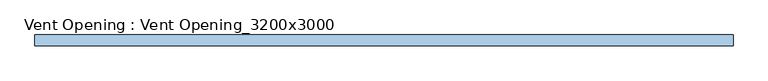
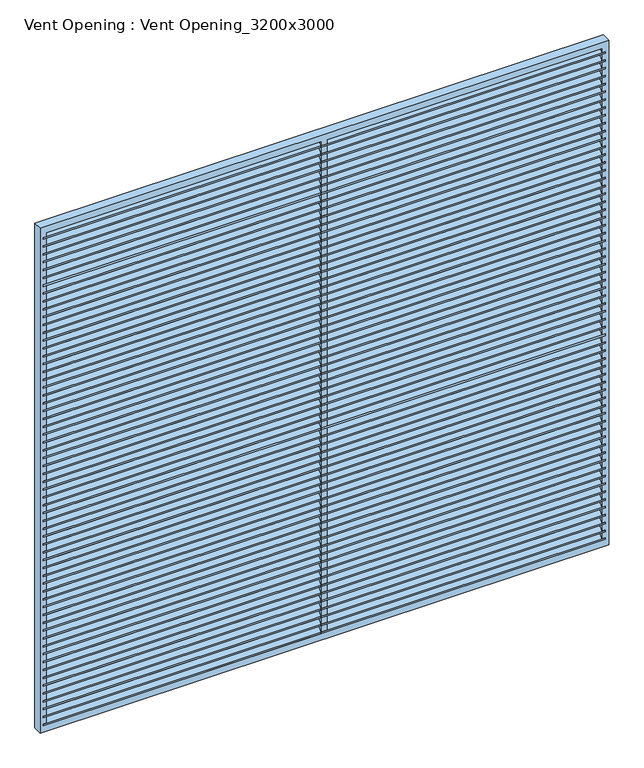
"""IFC4 building model written with IfcOpenShell, lengths in millimetres: window geometry, Vent Opening : Vent Opening_3200x3000."""

from ifc_helpers import new_model, si_unit, frame, origin, place, context, project, spatial, polyline, outline, extrude, source, transform, mapped, element, save


def vent_opening_vent_opening_3200x3000_4c487494(model_context):
    return source(origin(), model_context, "Body", "SweptSolid", [
        extrude(outline(polyline([(118.65, 3390.2900041), (118.65, 3381.309748), (93.65, 3406.309748), (68.65, 3381.309748), (68.65, 3390.2900041), (93.65, 3415.2900041), (118.65, 3390.2900041)])), frame((-1580.95, 0.0, 0.0), z_axis=(1.0, 0.0, 0.0), x_axis=(0.0, 1.0, 0.0)), (0.0, 0.0, 1.0), 3161.9),
        extrude(outline(polyline([(118.65, 3343.6800083), (118.65, 3334.6997521), (93.65, 3359.6997521), (68.65, 3334.6997521), (68.65, 3343.6800083), (93.65, 3368.6800083), (118.65, 3343.6800083)])), frame((-1580.95, 0.0, 0.0), z_axis=(1.0, 0.0, 0.0), x_axis=(0.0, 1.0, 0.0)), (0.0, 0.0, 1.0), 3161.9),
        extrude(outline(polyline([(118.65, 3297.0700124), (118.65, 3288.0897563), (93.65, 3313.0897563), (68.65, 3288.0897563), (68.65, 3297.0700124), (93.65, 3322.0700124), (118.65, 3297.0700124)])), frame((-1580.95, 0.0, 0.0), z_axis=(1.0, 0.0, 0.0), x_axis=(0.0, 1.0, 0.0)), (0.0, 0.0, 1.0), 3161.9),
        extrude(outline(polyline([(118.65, 3250.4600165), (118.65, 3241.4797604), (93.65, 3266.4797604), (68.65, 3241.4797604), (68.65, 3250.4600165), (93.65, 3275.4600165), (118.65, 3250.4600165)])), frame((-1580.95, 0.0, 0.0), z_axis=(1.0, 0.0, 0.0), x_axis=(0.0, 1.0, 0.0)), (0.0, 0.0, 1.0), 3161.9),
        extrude(outline(polyline([(118.65, 3203.8500207), (118.65, 3194.8697645), (93.65, 3219.8697645), (68.65, 3194.8697645), (68.65, 3203.8500207), (93.65, 3228.8500207), (118.65, 3203.8500207)])), frame((-1580.95, 0.0, 0.0), z_axis=(1.0, 0.0, 0.0), x_axis=(0.0, 1.0, 0.0)), (0.0, 0.0, 1.0), 3161.9),
        extrude(outline(polyline([(118.65, 3157.2400248), (118.65, 3148.2597687), (93.65, 3173.2597687), (68.65, 3148.2597687), (68.65, 3157.2400248), (93.65, 3182.2400248), (118.65, 3157.2400248)])), frame((-1580.95, 0.0, 0.0), z_axis=(1.0, 0.0, 0.0), x_axis=(0.0, 1.0, 0.0)), (0.0, 0.0, 1.0), 3161.9),
        extrude(outline(polyline([(118.65, 3110.6300289), (118.65, 3101.6497728), (93.65, 3126.6497728), (68.65, 3101.6497728), (68.65, 3110.6300289), (93.65, 3135.6300289), (118.65, 3110.6300289)])), frame((-1580.95, 0.0, 0.0), z_axis=(1.0, 0.0, 0.0), x_axis=(0.0, 1.0, 0.0)), (0.0, 0.0, 1.0), 3161.9),
        extrude(outline(polyline([(118.65, 3064.020033), (118.65, 3055.0397769), (93.65, 3080.0397769), (68.65, 3055.0397769), (68.65, 3064.020033), (93.65, 3089.020033), (118.65, 3064.020033)])), frame((-1580.95, 0.0, 0.0), z_axis=(1.0, 0.0, 0.0), x_axis=(0.0, 1.0, 0.0)), (0.0, 0.0, 1.0), 3161.9),
        extrude(outline(polyline([(118.65, 3017.4100372), (118.65, 3008.4297811), (93.65, 3033.4297811), (68.65, 3008.4297811), (68.65, 3017.4100372), (93.65, 3042.4100372), (118.65, 3017.4100372)])), frame((-1580.95, 0.0, 0.0), z_axis=(1.0, 0.0, 0.0), x_axis=(0.0, 1.0, 0.0)), (0.0, 0.0, 1.0), 3161.9),
        extrude(outline(polyline([(118.65, 2970.8000413), (118.65, 2961.8197852), (93.65, 2986.8197852), (68.65, 2961.8197852), (68.65, 2970.8000413), (93.65, 2995.8000413), (118.65, 2970.8000413)])), frame((-1580.95, 0.0, 0.0), z_axis=(1.0, 0.0, 0.0), x_axis=(0.0, 1.0, 0.0)), (0.0, 0.0, 1.0), 3161.9),
        extrude(outline(polyline([(118.65, 2924.1900454), (118.65, 2915.2097893), (93.65, 2940.2097893), (68.65, 2915.2097893), (68.65, 2924.1900454), (93.65, 2949.1900454), (118.65, 2924.1900454)])), frame((-1580.95, 0.0, 0.0), z_axis=(1.0, 0.0, 0.0), x_axis=(0.0, 1.0, 0.0)), (0.0, 0.0, 1.0), 3161.9),
        extrude(outline(polyline([(118.65, 2877.5800496), (118.65, 2868.5997935), (93.65, 2893.5997935), (68.65, 2868.5997935), (68.65, 2877.5800496), (93.65, 2902.5800496), (118.65, 2877.5800496)])), frame((-1580.95, 0.0, 0.0), z_axis=(1.0, 0.0, 0.0), x_axis=(0.0, 1.0, 0.0)), (0.0, 0.0, 1.0), 3161.9),
        extrude(outline(polyline([(118.65, 2830.9700537), (118.65, 2821.9897976), (93.65, 2846.9897976), (68.65, 2821.9897976), (68.65, 2830.9700537), (93.65, 2855.9700537), (118.65, 2830.9700537)])), frame((-1580.95, 0.0, 0.0), z_axis=(1.0, 0.0, 0.0), x_axis=(0.0, 1.0, 0.0)), (0.0, 0.0, 1.0), 3161.9),
        extrude(outline(polyline([(118.65, 2784.3600578), (118.65, 2775.3798017), (93.65, 2800.3798017), (68.65, 2775.3798017), (68.65, 2784.3600578), (93.65, 2809.3600578), (118.65, 2784.3600578)])), frame((-1580.95, 0.0, 0.0), z_axis=(1.0, 0.0, 0.0), x_axis=(0.0, 1.0, 0.0)), (0.0, 0.0, 1.0), 3161.9),
        extrude(outline(polyline([(118.65, 2737.750062), (118.65, 2728.7698058), (93.65, 2753.7698058), (68.65, 2728.7698058), (68.65, 2737.750062), (93.65, 2762.750062), (118.65, 2737.750062)])), frame((-1580.95, 0.0, 0.0), z_axis=(1.0, 0.0, 0.0), x_axis=(0.0, 1.0, 0.0)), (0.0, 0.0, 1.0), 3161.9),
        extrude(outline(polyline([(118.65, 2691.1400661), (118.65, 2682.15981), (93.65, 2707.15981), (68.65, 2682.15981), (68.65, 2691.1400661), (93.65, 2716.1400661), (118.65, 2691.1400661)])), frame((-1580.95, 0.0, 0.0), z_axis=(1.0, 0.0, 0.0), x_axis=(0.0, 1.0, 0.0)), (0.0, 0.0, 1.0), 3161.9),
        extrude(outline(polyline([(118.65, 2644.5300702), (118.65, 2635.5498141), (93.65, 2660.5498141), (68.65, 2635.5498141), (68.65, 2644.5300702), (93.65, 2669.5300702), (118.65, 2644.5300702)])), frame((-1580.95, 0.0, 0.0), z_axis=(1.0, 0.0, 0.0), x_axis=(0.0, 1.0, 0.0)), (0.0, 0.0, 1.0), 3161.9),
        extrude(outline(polyline([(118.65, 2597.9200744), (118.65, 2588.9398182), (93.65, 2613.9398182), (68.65, 2588.9398182), (68.65, 2597.9200744), (93.65, 2622.9200744), (118.65, 2597.9200744)])), frame((-1580.95, 0.0, 0.0), z_axis=(1.0, 0.0, 0.0), x_axis=(0.0, 1.0, 0.0)), (0.0, 0.0, 1.0), 3161.9),
        extrude(outline(polyline([(118.65, 2551.3100785), (118.65, 2542.3298224), (93.65, 2567.3298224), (68.65, 2542.3298224), (68.65, 2551.3100785), (93.65, 2576.3100785), (118.65, 2551.3100785)])), frame((-1580.95, 0.0, 0.0), z_axis=(1.0, 0.0, 0.0), x_axis=(0.0, 1.0, 0.0)), (0.0, 0.0, 1.0), 3161.9),
        extrude(outline(polyline([(118.65, 2504.7000826), (118.65, 2495.7198265), (93.65, 2520.7198265), (68.65, 2495.7198265), (68.65, 2504.7000826), (93.65, 2529.7000826), (118.65, 2504.7000826)])), frame((-1580.95, 0.0, 0.0), z_axis=(1.0, 0.0, 0.0), x_axis=(0.0, 1.0, 0.0)), (0.0, 0.0, 1.0), 3161.9),
        extrude(outline(polyline([(118.65, 2458.0900868), (118.65, 2449.1098306), (93.65, 2474.1098306), (68.65, 2449.1098306), (68.65, 2458.0900868), (93.65, 2483.0900868), (118.65, 2458.0900868)])), frame((-1580.95, 0.0, 0.0), z_axis=(1.0, 0.0, 0.0), x_axis=(0.0, 1.0, 0.0)), (0.0, 0.0, 1.0), 3161.9),
        extrude(outline(polyline([(118.65, 2411.4800909), (118.65, 2402.4998348), (93.65, 2427.4998348), (68.65, 2402.4998348), (68.65, 2411.4800909), (93.65, 2436.4800909), (118.65, 2411.4800909)])), frame((-1580.95, 0.0, 0.0), z_axis=(1.0, 0.0, 0.0), x_axis=(0.0, 1.0, 0.0)), (0.0, 0.0, 1.0), 3161.9),
        extrude(outline(polyline([(118.65, 2364.870095), (118.65, 2355.8898389), (93.65, 2380.8898389), (68.65, 2355.8898389), (68.65, 2364.870095), (93.65, 2389.870095), (118.65, 2364.870095)])), frame((-1580.95, 0.0, 0.0), z_axis=(1.0, 0.0, 0.0), x_axis=(0.0, 1.0, 0.0)), (0.0, 0.0, 1.0), 3161.9),
        extrude(outline(polyline([(118.65, 2318.2600991), (118.65, 2309.279843), (93.65, 2334.279843), (68.65, 2309.279843), (68.65, 2318.2600991), (93.65, 2343.2600991), (118.65, 2318.2600991)])), frame((-1580.95, 0.0, 0.0), z_axis=(1.0, 0.0, 0.0), x_axis=(0.0, 1.0, 0.0)), (0.0, 0.0, 1.0), 3161.9),
        extrude(outline(polyline([(118.65, 2271.6501033), (118.65, 2262.6698472), (93.65, 2287.6698472), (68.65, 2262.6698472), (68.65, 2271.6501033), (93.65, 2296.6501033), (118.65, 2271.6501033)])), frame((-1580.95, 0.0, 0.0), z_axis=(1.0, 0.0, 0.0), x_axis=(0.0, 1.0, 0.0)), (0.0, 0.0, 1.0), 3161.9),
        extrude(outline(polyline([(118.65, 2225.0401074), (118.65, 2216.0598513), (93.65, 2241.0598513), (68.65, 2216.0598513), (68.65, 2225.0401074), (93.65, 2250.0401074), (118.65, 2225.0401074)])), frame((-1580.95, 0.0, 0.0), z_axis=(1.0, 0.0, 0.0), x_axis=(0.0, 1.0, 0.0)), (0.0, 0.0, 1.0), 3161.9),
        extrude(outline(polyline([(118.65, 2178.4301115), (118.65, 2169.4498554), (93.65, 2194.4498554), (68.65, 2169.4498554), (68.65, 2178.4301115), (93.65, 2203.4301115), (118.65, 2178.4301115)])), frame((-1580.95, 0.0, 0.0), z_axis=(1.0, 0.0, 0.0), x_axis=(0.0, 1.0, 0.0)), (0.0, 0.0, 1.0), 3161.9),
        extrude(outline(polyline([(118.65, 2131.8201157), (118.65, 2122.8398595), (93.65, 2147.8398595), (68.65, 2122.8398595), (68.65, 2131.8201157), (93.65, 2156.8201157), (118.65, 2131.8201157)])), frame((-1580.95, 0.0, 0.0), z_axis=(1.0, 0.0, 0.0), x_axis=(0.0, 1.0, 0.0)), (0.0, 0.0, 1.0), 3161.9),
        extrude(outline(polyline([(118.65, 2085.2101198), (118.65, 2076.2298637), (93.65, 2101.2298637), (68.65, 2076.2298637), (68.65, 2085.2101198), (93.65, 2110.2101198), (118.65, 2085.2101198)])), frame((-1580.95, 0.0, 0.0), z_axis=(1.0, 0.0, 0.0), x_axis=(0.0, 1.0, 0.0)), (0.0, 0.0, 1.0), 3161.9),
        extrude(outline(polyline([(118.65, 2038.6001239), (118.65, 2029.6198678), (93.65, 2054.6198678), (68.65, 2029.6198678), (68.65, 2038.6001239), (93.65, 2063.6001239), (118.65, 2038.6001239)])), frame((-1580.95, 0.0, 0.0), z_axis=(1.0, 0.0, 0.0), x_axis=(0.0, 1.0, 0.0)), (0.0, 0.0, 1.0), 3161.9),
        extrude(outline(polyline([(118.65, 1991.9901281), (118.65, 1983.0098719), (93.65, 2008.0098719), (68.65, 1983.0098719), (68.65, 1991.9901281), (93.65, 2016.9901281), (118.65, 1991.9901281)])), frame((-1580.95, 0.0, 0.0), z_axis=(1.0, 0.0, 0.0), x_axis=(0.0, 1.0, 0.0)), (0.0, 0.0, 1.0), 3161.9),
        extrude(outline(polyline([(118.65, 1945.3801322), (118.65, 1936.3998761), (93.65, 1961.3998761), (68.65, 1936.3998761), (68.65, 1945.3801322), (93.65, 1970.3801322), (118.65, 1945.3801322)])), frame((-1580.95, 0.0, 0.0), z_axis=(1.0, 0.0, 0.0), x_axis=(0.0, 1.0, 0.0)), (0.0, 0.0, 1.0), 3161.9),
        extrude(outline(polyline([(118.65, 1898.7701363), (118.65, 1889.7898802), (93.65, 1914.7898802), (68.65, 1889.7898802), (68.65, 1898.7701363), (93.65, 1923.7701363), (118.65, 1898.7701363)])), frame((-1580.95, 0.0, 0.0), z_axis=(1.0, 0.0, 0.0), x_axis=(0.0, 1.0, 0.0)), (0.0, 0.0, 1.0), 3161.9),
        extrude(outline(polyline([(118.65, 1852.1601405), (118.65, 1843.1798843), (93.65, 1868.1798843), (68.65, 1843.1798843), (68.65, 1852.1601405), (93.65, 1877.1601405), (118.65, 1852.1601405)])), frame((-1580.95, 0.0, 0.0), z_axis=(1.0, 0.0, 0.0), x_axis=(0.0, 1.0, 0.0)), (0.0, 0.0, 1.0), 3161.9),
        extrude(outline(polyline([(118.65, 1805.5501446), (118.65, 1796.5698885), (93.65, 1821.5698885), (68.65, 1796.5698885), (68.65, 1805.5501446), (93.65, 1830.5501446), (118.65, 1805.5501446)])), frame((-1580.95, 0.0, 0.0), z_axis=(1.0, 0.0, 0.0), x_axis=(0.0, 1.0, 0.0)), (0.0, 0.0, 1.0), 3161.9),
        extrude(outline(polyline([(118.65, 1758.9401487), (118.65, 1749.9598926), (93.65, 1774.9598926), (68.65, 1749.9598926), (68.65, 1758.9401487), (93.65, 1783.9401487), (118.65, 1758.9401487)])), frame((-1580.95, 0.0, 0.0), z_axis=(1.0, 0.0, 0.0), x_axis=(0.0, 1.0, 0.0)), (0.0, 0.0, 1.0), 3161.9),
        extrude(outline(polyline([(118.65, 1712.3301528), (118.65, 1703.3498967), (93.65, 1728.3498967), (68.65, 1703.3498967), (68.65, 1712.3301528), (93.65, 1737.3301528), (118.65, 1712.3301528)])), frame((-1580.95, 0.0, 0.0), z_axis=(1.0, 0.0, 0.0), x_axis=(0.0, 1.0, 0.0)), (0.0, 0.0, 1.0), 3161.9),
        extrude(outline(polyline([(118.65, 1665.720157), (118.65, 1656.7399009), (93.65, 1681.7399009), (68.65, 1656.7399009), (68.65, 1665.720157), (93.65, 1690.720157), (118.65, 1665.720157)])), frame((-1580.95, 0.0, 0.0), z_axis=(1.0, 0.0, 0.0), x_axis=(0.0, 1.0, 0.0)), (0.0, 0.0, 1.0), 3161.9),
        extrude(outline(polyline([(118.65, 1619.1101611), (118.65, 1610.129905), (93.65, 1635.129905), (68.65, 1610.129905), (68.65, 1619.1101611), (93.65, 1644.1101611), (118.65, 1619.1101611)])), frame((-1580.95, 0.0, 0.0), z_axis=(1.0, 0.0, 0.0), x_axis=(0.0, 1.0, 0.0)), (0.0, 0.0, 1.0), 3161.9),
        extrude(outline(polyline([(118.65, 1572.5001652), (118.65, 1563.5199091), (93.65, 1588.5199091), (68.65, 1563.5199091), (68.65, 1572.5001652), (93.65, 1597.5001652), (118.65, 1572.5001652)])), frame((-1580.95, 0.0, 0.0), z_axis=(1.0, 0.0, 0.0), x_axis=(0.0, 1.0, 0.0)), (0.0, 0.0, 1.0), 3161.9),
        extrude(outline(polyline([(118.65, 1525.8901694), (118.65, 1516.9099132), (93.65, 1541.9099132), (68.65, 1516.9099132), (68.65, 1525.8901694), (93.65, 1550.8901694), (118.65, 1525.8901694)])), frame((-1580.95, 0.0, 0.0), z_axis=(1.0, 0.0, 0.0), x_axis=(0.0, 1.0, 0.0)), (0.0, 0.0, 1.0), 3161.9),
        extrude(outline(polyline([(118.65, 1479.2801735), (118.65, 1470.2999174), (93.65, 1495.2999174), (68.65, 1470.2999174), (68.65, 1479.2801735), (93.65, 1504.2801735), (118.65, 1479.2801735)])), frame((-1580.95, 0.0, 0.0), z_axis=(1.0, 0.0, 0.0), x_axis=(0.0, 1.0, 0.0)), (0.0, 0.0, 1.0), 3161.9),
        extrude(outline(polyline([(118.65, 1432.6701776), (118.65, 1423.6899215), (93.65, 1448.6899215), (68.65, 1423.6899215), (68.65, 1432.6701776), (93.65, 1457.6701776), (118.65, 1432.6701776)])), frame((-1580.95, 0.0, 0.0), z_axis=(1.0, 0.0, 0.0), x_axis=(0.0, 1.0, 0.0)), (0.0, 0.0, 1.0), 3161.9),
        extrude(outline(polyline([(118.65, 1386.0601818), (118.65, 1377.0799256), (93.65, 1402.0799256), (68.65, 1377.0799256), (68.65, 1386.0601818), (93.65, 1411.0601818), (118.65, 1386.0601818)])), frame((-1580.95, 0.0, 0.0), z_axis=(1.0, 0.0, 0.0), x_axis=(0.0, 1.0, 0.0)), (0.0, 0.0, 1.0), 3161.9),
        extrude(outline(polyline([(118.65, 1339.4501859), (118.65, 1330.4699298), (93.65, 1355.4699298), (68.65, 1330.4699298), (68.65, 1339.4501859), (93.65, 1364.4501859), (118.65, 1339.4501859)])), frame((-1580.95, 0.0, 0.0), z_axis=(1.0, 0.0, 0.0), x_axis=(0.0, 1.0, 0.0)), (0.0, 0.0, 1.0), 3161.9),
        extrude(outline(polyline([(118.65, 1292.84019), (118.65, 1283.8599339), (93.65, 1308.8599339), (68.65, 1283.8599339), (68.65, 1292.84019), (93.65, 1317.84019), (118.65, 1292.84019)])), frame((-1580.95, 0.0, 0.0), z_axis=(1.0, 0.0, 0.0), x_axis=(0.0, 1.0, 0.0)), (0.0, 0.0, 1.0), 3161.9),
        extrude(outline(polyline([(118.65, 1246.2301942), (118.65, 1237.249938), (93.65, 1262.249938), (68.65, 1237.249938), (68.65, 1246.2301942), (93.65, 1271.2301942), (118.65, 1246.2301942)])), frame((-1580.95, 0.0, 0.0), z_axis=(1.0, 0.0, 0.0), x_axis=(0.0, 1.0, 0.0)), (0.0, 0.0, 1.0), 3161.9),
        extrude(outline(polyline([(118.65, 1199.6201983), (118.65, 1190.6399422), (93.65, 1215.6399422), (68.65, 1190.6399422), (68.65, 1199.6201983), (93.65, 1224.6201983), (118.65, 1199.6201983)])), frame((-1580.95, 0.0, 0.0), z_axis=(1.0, 0.0, 0.0), x_axis=(0.0, 1.0, 0.0)), (0.0, 0.0, 1.0), 3161.9),
        extrude(outline(polyline([(118.65, 1153.0102024), (118.65, 1144.0299463), (93.65, 1169.0299463), (68.65, 1144.0299463), (68.65, 1153.0102024), (93.65, 1178.0102024), (118.65, 1153.0102024)])), frame((-1580.95, 0.0, 0.0), z_axis=(1.0, 0.0, 0.0), x_axis=(0.0, 1.0, 0.0)), (0.0, 0.0, 1.0), 3161.9),
        extrude(outline(polyline([(118.65, 1106.4002065), (118.65, 1097.4199504), (93.65, 1122.4199504), (68.65, 1097.4199504), (68.65, 1106.4002065), (93.65, 1131.4002065), (118.65, 1106.4002065)])), frame((-1580.95, 0.0, 0.0), z_axis=(1.0, 0.0, 0.0), x_axis=(0.0, 1.0, 0.0)), (0.0, 0.0, 1.0), 3161.9),
        extrude(outline(polyline([(118.65, 1059.7902107), (118.65, 1050.8099546), (93.65, 1075.8099546), (68.65, 1050.8099546), (68.65, 1059.7902107), (93.65, 1084.7902107), (118.65, 1059.7902107)])), frame((-1580.95, 0.0, 0.0), z_axis=(1.0, 0.0, 0.0), x_axis=(0.0, 1.0, 0.0)), (0.0, 0.0, 1.0), 3161.9),
        extrude(outline(polyline([(118.65, 1013.1802148), (118.65, 1004.1999587), (93.65, 1029.1999587), (68.65, 1004.1999587), (68.65, 1013.1802148), (93.65, 1038.1802148), (118.65, 1013.1802148)])), frame((-1580.95, 0.0, 0.0), z_axis=(1.0, 0.0, 0.0), x_axis=(0.0, 1.0, 0.0)), (0.0, 0.0, 1.0), 3161.9),
        extrude(outline(polyline([(118.65, 966.5702189), (118.65, 957.5899628), (93.65, 982.5899628), (68.65, 957.5899628), (68.65, 966.5702189), (93.65, 991.5702189), (118.65, 966.5702189)])), frame((-1580.95, 0.0, 0.0), z_axis=(1.0, 0.0, 0.0), x_axis=(0.0, 1.0, 0.0)), (0.0, 0.0, 1.0), 3161.9),
        extrude(outline(polyline([(118.65, 919.9602231), (118.65, 910.979967), (93.65, 935.979967), (68.65, 910.979967), (68.65, 919.9602231), (93.65, 944.9602231), (118.65, 919.9602231)])), frame((-1580.95, 0.0, 0.0), z_axis=(1.0, 0.0, 0.0), x_axis=(0.0, 1.0, 0.0)), (0.0, 0.0, 1.0), 3161.9),
        extrude(outline(polyline([(118.65, 873.3502272), (118.65, 864.3699711), (93.65, 889.3699711), (68.65, 864.3699711), (68.65, 873.3502272), (93.65, 898.3502272), (118.65, 873.3502272)])), frame((-1580.95, 0.0, 0.0), z_axis=(1.0, 0.0, 0.0), x_axis=(0.0, 1.0, 0.0)), (0.0, 0.0, 1.0), 3161.9),
        extrude(outline(polyline([(118.65, 826.7402313), (118.65, 817.7599752), (93.65, 842.7599752), (68.65, 817.7599752), (68.65, 826.7402313), (93.65, 851.7402313), (118.65, 826.7402313)])), frame((-1580.95, 0.0, 0.0), z_axis=(1.0, 0.0, 0.0), x_axis=(0.0, 1.0, 0.0)), (0.0, 0.0, 1.0), 3161.9),
        extrude(outline(polyline([(118.65, 780.1302355), (118.65, 771.1499793), (93.65, 796.1499793), (68.65, 771.1499793), (68.65, 780.1302355), (93.65, 805.1302355), (118.65, 780.1302355)])), frame((-1580.95, 0.0, 0.0), z_axis=(1.0, 0.0, 0.0), x_axis=(0.0, 1.0, 0.0)), (0.0, 0.0, 1.0), 3161.9),
        extrude(outline(polyline([(118.65, 733.5202396), (118.65, 724.5399835), (93.65, 749.5399835), (68.65, 724.5399835), (68.65, 733.5202396), (93.65, 758.5202396), (118.65, 733.5202396)])), frame((-1580.95, 0.0, 0.0), z_axis=(1.0, 0.0, 0.0), x_axis=(0.0, 1.0, 0.0)), (0.0, 0.0, 1.0), 3161.9),
        extrude(outline(polyline([(118.65, 686.9102437), (118.65, 677.9299876), (93.65, 702.9299876), (68.65, 677.9299876), (68.65, 686.9102437), (93.65, 711.9102437), (118.65, 686.9102437)])), frame((-1580.95, 0.0, 0.0), z_axis=(1.0, 0.0, 0.0), x_axis=(0.0, 1.0, 0.0)), (0.0, 0.0, 1.0), 3161.9),
        extrude(outline(polyline([(118.65, 640.3002479), (118.65, 631.3199917), (93.65, 656.3199917), (68.65, 631.3199917), (68.65, 640.3002479), (93.65, 665.3002479), (118.65, 640.3002479)])), frame((-1580.95, 0.0, 0.0), z_axis=(1.0, 0.0, 0.0), x_axis=(0.0, 1.0, 0.0)), (0.0, 0.0, 1.0), 3161.9),
        extrude(outline(polyline([(118.65, 593.690252), (118.65, 584.7099959), (93.65, 609.7099959), (68.65, 584.7099959), (68.65, 593.690252), (93.65, 618.690252), (118.65, 593.690252)])), frame((-1580.95, 0.0, 0.0), z_axis=(1.0, 0.0, 0.0), x_axis=(0.0, 1.0, 0.0)), (0.0, 0.0, 1.0), 3161.9),
        extrude(outline(polyline([(118.65, 3436.9), (118.65, 3427.9197439), (93.65, 3452.9197439), (68.65, 3427.9197439), (68.65, 3436.9), (93.65, 3461.9), (118.65, 3436.9)])), frame((-1580.95, 0.0, 0.0), z_axis=(1.0, 0.0, 0.0), x_axis=(0.0, 1.0, 0.0)), (0.0, 0.0, 1.0), 3161.9),
        extrude(outline(polyline([(118.65, 547.0802561), (118.65, 538.1), (93.65, 563.1), (68.65, 538.1), (68.65, 547.0802561), (93.65, 572.0802561), (118.65, 547.0802561)])), frame((-1580.95, 0.0, 0.0), z_axis=(1.0, 0.0, 0.0), x_axis=(0.0, 1.0, 0.0)), (0.0, 0.0, 1.0), 3161.9),
        extrude(outline(polyline([(3500.0, -1600.0), (500.0, -1600.0), (500.0, 1600.0), (3500.0, 1600.0), (3500.0, -1600.0)]), holes=[polyline([(538.1, -1561.9), (3461.9, -1561.9), (3461.9, -19.05), (538.1, -19.05), (538.1, -1561.9)]), polyline([(3461.9, 19.05), (3461.9, 1561.9), (538.1, 1561.9), (538.1, 19.05), (3461.9, 19.05)])]), frame((0.0, 68.65, 0.0), z_axis=(0.0, 1.0, 0.0), x_axis=(0.0, 0.0, 1.0)), (0.0, 0.0, 1.0), 50.0),
    ])


if __name__ == "__main__":
    model = new_model("IFC4")
    model_context = context("Model", 3, world=origin())
    ifc_project = project(units=[si_unit("LENGTHUNIT", "METRE", prefix="MILLI")], contexts=[model_context])
    site = spatial("IfcSite", under=ifc_project)
    building = spatial("IfcBuilding", under=site)
    placement = place(None, origin())
    vent_opening_vent_opening_3200x3000_shape = vent_opening_vent_opening_3200x3000_4c487494(model_context)
    element("IfcWindow", 1, ObjectType="Vent Opening : Vent Opening_3200x3000", at=placement, inside=building, context=model_context, shape_type="MappedRepresentation", body=[
        mapped(vent_opening_vent_opening_3200x3000_shape, transform((0.0, 0.0, 0.0), x_axis=(1.0, 0.0, 0.0), y_axis=(0.0, 1.0, 0.0), z_axis=(0.0, 0.0, 1.0))),
    ])
    save(model, "model.ifc")

# Revit data of these elements
# Type "Vent Opening : Vent Opening_3200x3000"
#   Type Mark = "299"
#   Assembly Code = "B20"
#   Visual Light Transmittance = 0.9
#   Solar Heat Gain Coefficient = 0.78
#   Max Height = 2991.056 mm
#   Height = 3000 mm
#   Heat Transfer Coefficient (U) = 3.6886 W/(m²·K)
#   Blade Width [instance default] = 3161.9 mm
#   Blade Vertical Thickness = 8.98 mm
#   Blade Thickness = 6.35 mm
#   Blade Spacing = 38.1 mm
#   Blade Height = 33.98 mm
#   Blade Depth = 50 mm
#   Blade Angle = 45.00°
#   Default Sill Height = 500 mm
#   Trim Projection_Exterior = 12.7 mm
#   Trim Projection_Interior = 12.7 mm
#   Trim Width_Exterior = 38.1 mm
#   Trim Width_Interior = 38.1 mm
#   Width = 3200 mm
#   Max Blade Count = 63
#   Define Thermal Properties by = 1
#   Blade Count = 63
#   Frame Material = Birch
#   Louver Material = Birch
#   Trim Exterior Material = Birch
#   Trim Interior Material = Birch
#   Thermal Resistance (R) = 0
#   Construction Type Id = ""
#   Wall Closure = (empty or 0)
#   Analytic Construction = (empty or 0)
# Element 1 (IfcWindow, "Vent Opening : Vent Opening_3200x3000")
#   Materials on its faces: "00_Metal_Steel"
# Materials
#   "Birch": class "Wood", colour RGB 224 178 126, transparency 0, Description = "Betula Alleghaniensis", Cost = 0
#   "00_Metal_Steel": class "Metal", colour RGB 148 148 148, transparency 0, Description = "Steel", Cost = 0, Image = Doors - Windows.Glazed Curtain Walls.Stainless Steel Curtain Wall.jpg
